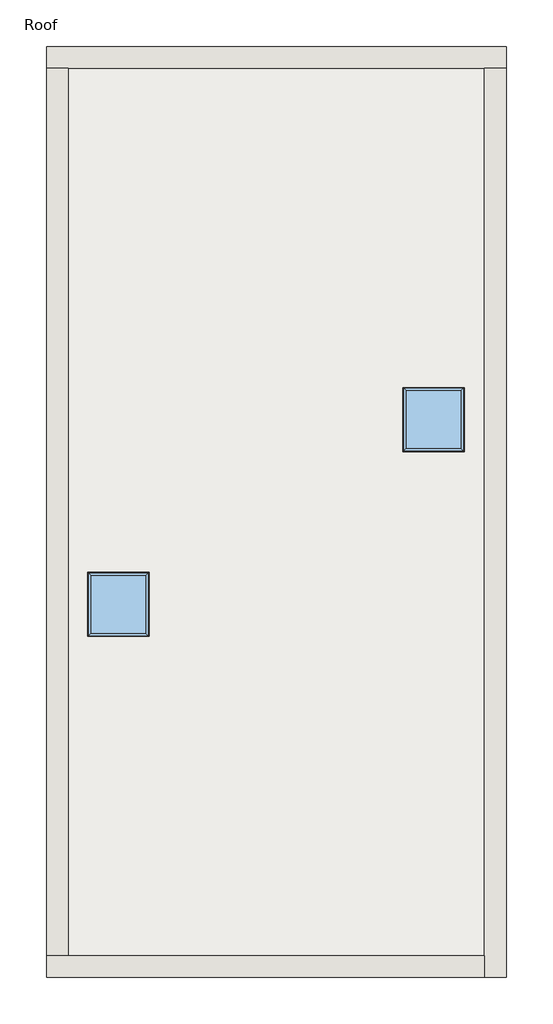
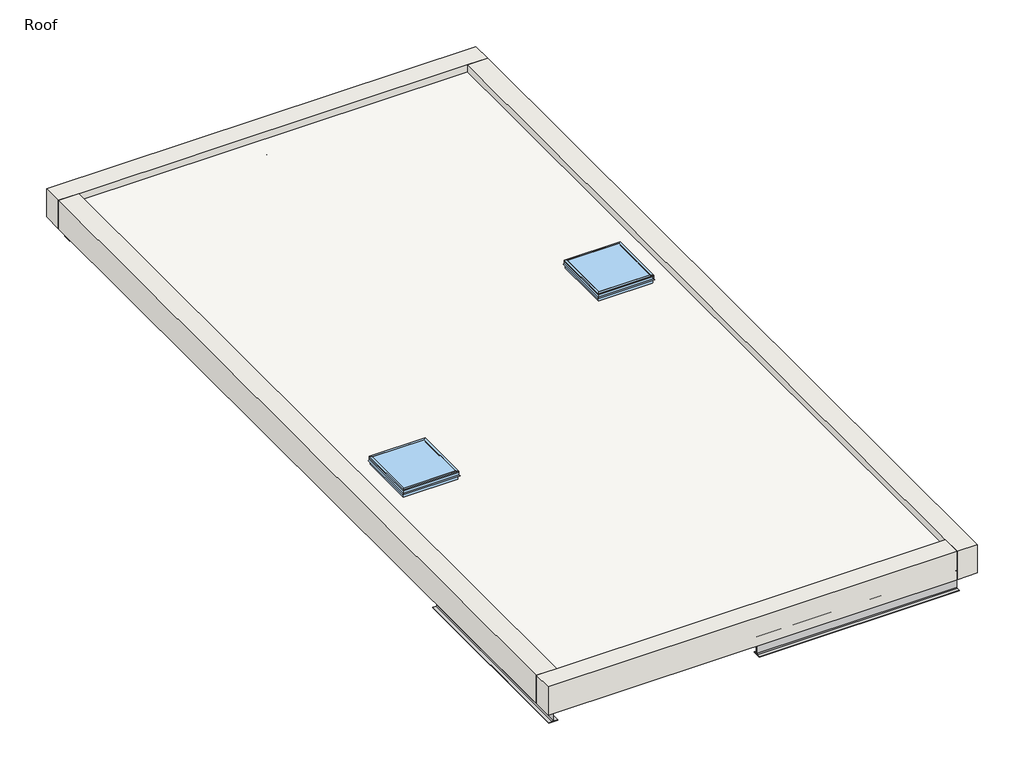
# One storey: 4 beams, 4 walls, 2 windows, 1 roof.
"""IFC4 building model written with IfcOpenShell, lengths in millimetres."""

import ifcopenshell
import ifcopenshell.guid

model = None  # the IFC model being written
_history = None  # IfcOwnerHistory: only IFC2X3 demands one
_inside = {}  # id of a spatial element -> (the spatial element, [elements in it])
_under = {}  # id of a project, library or spatial element -> (it, [spatial elements below it])
_declared = {}  # id of a project -> (the project, [libraries it declares])
_typed = {}  # id of a type object -> (the type object, [elements of that type])
_made_of = {}  # id of a material, layer set ... -> (it, [elements and type objects made of it])


def new_model(schema):
    """Start an empty IFC model of exactly this schema.

    Asked for "IFC4X3", IfcOpenShell would pick the latest addendum, in which some entities
    have other attributes; the version numbers below select the first issue.
    IFC2X3 requires an IfcOwnerHistory on every rooted entity: one is made here for all.
    """
    global model, _history
    if schema == "IFC4X3":
        model = ifcopenshell.file(schema_version=(4, 3, 0, 0))
    else:
        model = ifcopenshell.file(schema=schema)
    _inside.clear()
    _under.clear()
    _declared.clear()
    _typed.clear()
    _made_of.clear()
    _history = None
    if model.schema == "IFC2X3":
        org = make("IfcOrganization", Name="unknown")
        user = make(
            "IfcPersonAndOrganization",
            ThePerson=make("IfcPerson", FamilyName="unknown"),
            TheOrganization=org,
        )
        app = make(
            "IfcApplication",
            ApplicationDeveloper=org,
            Version="unknown",
            ApplicationFullName="unknown",
            ApplicationIdentifier="unknown",
        )
        _history = make(
            "IfcOwnerHistory",
            OwningUser=user,
            OwningApplication=app,
            ChangeAction="ADDED",
            CreationDate=0,
        )
    return model


def make(cls, **values):
    """One entity of the class cls with the attributes given. An attribute that is None is left unset."""
    return model.create_entity(
        cls, **{name: value for name, value in values.items() if value is not None}
    )


def rooted(cls, **values):
    """An entity with a GlobalId (a new one), such as an element, a storey or a relation."""
    return make(cls, GlobalId=ifcopenshell.guid.new(), OwnerHistory=_history, **values)


def si_unit(unit_type, name, prefix=None):
    """IfcSIUnit, for example si_unit("LENGTHUNIT", "METRE", prefix="MILLI")."""
    return make("IfcSIUnit", UnitType=unit_type, Prefix=prefix, Name=name)


def assignment(units):
    """IfcUnitAssignment: the units of a project."""
    return None if units is None else make("IfcUnitAssignment", Units=units)


def point(xyz):
    """IfcCartesianPoint."""
    return None if xyz is None else make("IfcCartesianPoint", Coordinates=xyz)


def direction(xyz):
    """IfcDirection."""
    return None if xyz is None else make("IfcDirection", DirectionRatios=xyz)


def frame(location, z_axis=None, x_axis=None):
    """IfcAxis2Placement3D, a coordinate frame: its origin and axes. An axis left out is left unset."""
    return make(
        "IfcAxis2Placement3D",
        Location=point(location),
        Axis=direction(z_axis),
        RefDirection=direction(x_axis),
    )


def frame_2d(location, x_axis=None):
    """IfcAxis2Placement2D, a coordinate frame in the plane: its origin and x axis."""
    return make(
        "IfcAxis2Placement2D", Location=point(location), RefDirection=direction(x_axis)
    )


def origin():
    """The frame at (0, 0, 0) with its axes left unset."""
    return frame((0.0, 0.0, 0.0))


def place(relative_to, where):
    """IfcLocalPlacement: puts the frame where relative to a parent placement (None: the world)."""
    return make(
        "IfcLocalPlacement", PlacementRelTo=relative_to, RelativePlacement=where
    )


def context(
    kind, dimensions, precision=None, world=None, true_north=None, identifier=None
):
    """IfcGeometricRepresentationContext, for example the 3D "Model" context."""
    return make(
        "IfcGeometricRepresentationContext",
        ContextIdentifier=identifier,
        ContextType=kind,
        CoordinateSpaceDimension=dimensions,
        Precision=precision,
        WorldCoordinateSystem=world,
        TrueNorth=true_north,
    )


def project(units=None, contexts=None):
    """IfcProject with its units and contexts."""
    return rooted(
        "IfcProject",
        Name="project",
        RepresentationContexts=contexts,
        UnitsInContext=assignment(units),
    )


def spatial(cls, under=None, at=None, **own):
    """A site, building, storey or space (cls), placed at a placement, below another one or the project."""
    s = rooted(cls, ObjectPlacement=at, **own)
    if under is not None:
        _under.setdefault(under.id(), (under, []))[1].append(s)
    return s


def polyline(points):
    """IfcPolyline through the points."""
    return make("IfcPolyline", Points=[point(p) for p in points])


def circle_curve(where, radius):
    """IfcCircle in the frame where."""
    return make("IfcCircle", Position=where, Radius=radius)


def trimmed(basis, trim1, trim2, sense, master):
    """IfcTrimmedCurve: the piece of a basis curve between two trims."""
    return make(
        "IfcTrimmedCurve",
        BasisCurve=basis,
        Trim1=trim1,
        Trim2=trim2,
        SenseAgreement=sense,
        MasterRepresentation=master,
    )


def segment(curve, same_sense, transition):
    """IfcCompositeCurveSegment."""
    return make(
        "IfcCompositeCurveSegment",
        Transition=transition,
        SameSense=same_sense,
        ParentCurve=curve,
    )


def composite_curve(segments, self_intersect=None):
    """IfcCompositeCurve: segments joined end to end."""
    return make("IfcCompositeCurve", Segments=segments, SelfIntersect=self_intersect)


def outline(outer, holes=None, kind="AREA"):
    """IfcArbitraryClosedProfileDef: a profile drawn as a closed curve; with holes, ...WithVoids."""
    if holes is None:
        return make("IfcArbitraryClosedProfileDef", ProfileType=kind, OuterCurve=outer)
    return make(
        "IfcArbitraryProfileDefWithVoids",
        ProfileType=kind,
        OuterCurve=outer,
        InnerCurves=holes,
    )


def extrude(swept, where, along, depth):
    """IfcExtrudedAreaSolid: the profile swept, set in the frame where, extruded along a direction by depth."""
    return make(
        "IfcExtrudedAreaSolid",
        SweptArea=swept,
        Position=where,
        ExtrudedDirection=direction(along),
        Depth=depth,
    )


def faces_of(points, faces, orient=None, outer=None):
    """IfcFace entities. A face is a list of loops; a loop is a list of indices into points, from 0.

    orient and outer hold one flag for each loop. By default every Orientation is true, the
    first loop of a face is its IfcFaceOuterBound and the others are IfcFaceBound.
    """
    made = []
    for i, loops in enumerate(faces):
        bounds = []
        for j, loop in enumerate(loops):
            is_outer = j == 0 if outer is None else outer[i][j]
            bounds.append(
                make(
                    "IfcFaceOuterBound" if is_outer else "IfcFaceBound",
                    Bound=make("IfcPolyLoop", Polygon=[points[k] for k in loop]),
                    Orientation=True if orient is None else orient[i][j],
                )
            )
        made.append(make("IfcFace", Bounds=bounds))
    return made


def faceted_brep(points, faces, orient=None, outer=None, voids=None):
    """IfcFacetedBrep: a solid bounded by flat faces; with voids (closed shells), ...WithVoids."""
    shared = [point(p) for p in points]
    hull = make("IfcClosedShell", CfsFaces=faces_of(shared, faces, orient, outer))
    if voids is None:
        return make("IfcFacetedBrep", Outer=hull)
    return make(
        "IfcFacetedBrepWithVoids",
        Outer=hull,
        Voids=[
            make(cls, CfsFaces=faces_of(shared, fs, o, b)) for cls, fs, o, b in voids
        ],
    )


def shape(context_of_items, identifier, shape_type, items):
    """IfcShapeRepresentation: the items that make up one representation, for example the "Body"."""
    return make(
        "IfcShapeRepresentation",
        ContextOfItems=context_of_items,
        RepresentationIdentifier=identifier,
        RepresentationType=shape_type,
        Items=items,
    )


def source(mapping_origin, context_of_items, identifier, shape_type, items):
    """IfcRepresentationMap: a shape defined once, which mapped items show again and again."""
    return make(
        "IfcRepresentationMap",
        MappingOrigin=mapping_origin,
        MappedRepresentation=shape(context_of_items, identifier, shape_type, items),
    )


def transform(
    local_origin,
    x_axis=None,
    y_axis=None,
    z_axis=None,
    scale=None,
    scale2=None,
    scale3=None,
    uniform=True,
):
    """IfcCartesianTransformationOperator3D, or its non-uniform kind. x_axis, y_axis, z_axis: its Axis1, 2, 3."""
    if uniform:
        return make(
            "IfcCartesianTransformationOperator3D",
            Axis1=direction(x_axis),
            Axis2=direction(y_axis),
            LocalOrigin=point(local_origin),
            Scale=scale,
            Axis3=direction(z_axis),
        )
    return make(
        "IfcCartesianTransformationOperator3DnonUniform",
        Axis1=direction(x_axis),
        Axis2=direction(y_axis),
        LocalOrigin=point(local_origin),
        Scale=scale,
        Axis3=direction(z_axis),
        Scale2=scale2,
        Scale3=scale3,
    )


def mapped(mapping_source, mapping_target):
    """IfcMappedItem: shows the shape of a source again, moved by a transform."""
    return make(
        "IfcMappedItem", MappingSource=mapping_source, MappingTarget=mapping_target
    )


def made_of(thing, what):
    """Note that an element or type object is made of a material, layer set ...; save() writes the relation."""
    if what is not None:
        _made_of.setdefault(what.id(), (what, []))[1].append(thing)
    return thing


def element(
    cls,
    number,
    at=None,
    inside=None,
    cuts=None,
    type_object=None,
    material=None,
    context=None,
    identifier="Body",
    shape_type=None,
    held_by="IfcProductDefinitionShape",
    body=None,
    shapes=None,
    **own,
):
    """One element of the class cls, such as IfcWall. Its Tag is "e" and its number.

    at: its placement. inside: the storey or other place that contains it. cuts: it is an
    opening in that element (IfcRelVoidsElement). A single representation is given by context,
    identifier, shape_type and body (its items); several are given by shapes. held_by: the class
    of the entity that holds the representations. save() writes the other relations.
    """
    e = rooted(cls, Tag="e%d" % number, ObjectPlacement=at, **own)
    if body is not None:
        shapes = [shape(context, identifier, shape_type, body)]
    if shapes is not None:
        e.Representation = make(held_by, Representations=shapes)
    if inside is not None:
        _inside.setdefault(inside.id(), (inside, []))[1].append(e)
    if cuts is not None:
        rooted(
            "IfcRelVoidsElement", RelatingBuildingElement=cuts, RelatedOpeningElement=e
        )
    if type_object is not None:
        _typed.setdefault(type_object.id(), (type_object, []))[1].append(e)
    return made_of(e, material)


def aggregate(whole, parts):
    """IfcRelAggregates: a whole, such as a stair, and the parts it consists of."""
    return rooted("IfcRelAggregates", RelatingObject=whole, RelatedObjects=parts)


def save(model, path):
    """Write the relations noted so far, then the file.

    IfcRelAggregates (storeys below a building ...), IfcRelContainedInSpatialStructure (elements
    in a storey), IfcRelDefinesByType, IfcRelAssociatesMaterial and IfcRelDeclares: one each for
    every whole, place, type object, material and project.
    """
    for whole, parts in _under.values():
        aggregate(whole, parts)
    for where, things in _inside.values():
        rooted(
            "IfcRelContainedInSpatialStructure",
            RelatedElements=things,
            RelatingStructure=where,
        )
    for kind, things in _typed.values():
        rooted("IfcRelDefinesByType", RelatedObjects=things, RelatingType=kind)
    for what, things in _made_of.values():
        rooted("IfcRelAssociatesMaterial", RelatedObjects=things, RelatingMaterial=what)
    for by, libraries in _declared.values():
        rooted("IfcRelDeclares", RelatingContext=by, RelatedDefinitions=libraries)
    model.write(path)


def w410x60_ca7ba955(model_context):
    return source(origin(), model_context, "Body", "SweptSolid", [
        extrude(outline(composite_curve([segment(polyline([(89.0, -190.7), (89.0, -203.5), (-89.0, -203.5), (-89.0, -190.7), (-21.05, -190.7)]), True, "CONTINUOUS"), segment(trimmed(circle_curve(frame_2d((-21.05, -173.5)), 17.2), [point((-21.05, -190.7))], [point((-3.85, -173.5))], True, "CARTESIAN"), True, "CONTINUOUS"), segment(polyline([(-3.85, -173.5), (-3.85, 173.5)]), True, "CONTINUOUS"), segment(trimmed(circle_curve(frame_2d((-21.05, 173.5)), 17.2), [point((-3.85, 173.5))], [point((-21.05, 190.7))], True, "CARTESIAN"), True, "CONTINUOUS"), segment(polyline([(-21.05, 190.7), (-89.0, 190.7), (-89.0, 203.5), (89.0, 203.5), (89.0, 190.7), (21.05, 190.7)]), True, "CONTINUOUS"), segment(trimmed(circle_curve(frame_2d((21.05, 173.5)), 17.2), [point((21.05, 190.7))], [point((3.85, 173.5))], True, "CARTESIAN"), True, "CONTINUOUS"), segment(polyline([(3.85, 173.5), (3.85, -173.5)]), True, "CONTINUOUS"), segment(trimmed(circle_curve(frame_2d((21.05, -173.5)), 17.2), [point((3.85, -173.5))], [point((21.05, -190.7))], True, "CARTESIAN"), True, "CONTINUOUS"), segment(polyline([(21.05, -190.7), (89.0, -190.7)]), True, "CONTINUOUS")], self_intersect=False)), frame((-2050.0, 0.0, 0.0), z_axis=(1.0, 0.0, 0.0), x_axis=(0.0, 1.0, 0.0)), (0.0, 0.0, 1.0), 4100.0),
    ])


def w410x60_6fd633e1(model_context):
    return source(origin(), model_context, "Body", "SweptSolid", [
        extrude(outline(composite_curve([segment(polyline([(89.0, -190.7), (89.0, -203.5), (-89.0, -203.5), (-89.0, -190.7), (-21.05, -190.7)]), True, "CONTINUOUS"), segment(trimmed(circle_curve(frame_2d((-21.05, -173.5)), 17.2), [point((-21.05, -190.7))], [point((-3.85, -173.5))], True, "CARTESIAN"), True, "CONTINUOUS"), segment(polyline([(-3.85, -173.5), (-3.85, 173.5)]), True, "CONTINUOUS"), segment(trimmed(circle_curve(frame_2d((-21.05, 173.5)), 17.2), [point((-3.85, 173.5))], [point((-21.05, 190.7))], True, "CARTESIAN"), True, "CONTINUOUS"), segment(polyline([(-21.05, 190.7), (-89.0, 190.7), (-89.0, 203.5), (89.0, 203.5), (89.0, 190.7), (21.05, 190.7)]), True, "CONTINUOUS"), segment(trimmed(circle_curve(frame_2d((21.05, 173.5)), 17.2), [point((21.05, 190.7))], [point((3.85, 173.5))], True, "CARTESIAN"), True, "CONTINUOUS"), segment(polyline([(3.85, 173.5), (3.85, -173.5)]), True, "CONTINUOUS"), segment(trimmed(circle_curve(frame_2d((21.05, -173.5)), 17.2), [point((3.85, -173.5))], [point((21.05, -190.7))], True, "CARTESIAN"), True, "CONTINUOUS"), segment(polyline([(21.05, -190.7), (89.0, -190.7)]), True, "CONTINUOUS")], self_intersect=False)), frame((-2060.6399643, 0.0, 0.0), z_axis=(1.0, 0.0, 0.0), x_axis=(0.0, 1.0, 0.0)), (0.0, 0.0, 1.0), 4121.2799286),
    ])


def m_skylight_1180_x_1170mm_371bb450(model_context):
    return source(origin(), model_context, "Body", "SolidModel", [
        faceted_brep([(254.440073, 370.1040988, 4267.0), (279.840073, 395.5040988, 4267.0), (279.840073, -774.4959012, 4267.0), (254.440073, -749.0959012, 4267.0), (254.440073, 370.1040988, 4292.4), (254.440073, -749.0959012, 4292.4), (292.540073, 408.2040988, 4292.4), (292.540073, -787.1959012, 4292.4), (292.540073, 408.2040988, 4267.0), (292.540073, -787.1959012, 4267.0), (292.540073, 408.2040988, 4216.2), (292.540073, -787.1959012, 4216.2), (307.1089145, 422.7729403, 4195.3935381), (307.1089145, -801.7647427, 4195.3935381), (301.907299, 417.5713248, 4191.7513277), (301.907299, -796.5631272, 4191.7513277), (286.190073, 401.8540988, 4214.1978527), (286.190073, -780.8459012, 4214.1978527), (286.190073, 401.8540988, 4267.0), (286.190073, -780.8459012, 4267.0), (-838.159927, -774.4959012, 4267.0), (-812.759927, -749.0959012, 4267.0), (-812.759927, -749.0959012, 4292.4), (-850.859927, -787.1959012, 4292.4), (-850.859927, -787.1959012, 4267.0), (-850.859927, -787.1959012, 4216.2), (-865.4287685, -801.7647427, 4195.3935381), (-860.227153, -796.5631272, 4191.7513277), (-844.509927, -780.8459012, 4214.1978527), (-844.509927, -780.8459012, 4267.0), (-838.159927, 395.5040988, 4267.0), (-812.759927, 370.1040988, 4267.0), (-812.759927, 370.1040988, 4292.4), (-850.859927, 408.2040988, 4292.4), (-850.859927, 408.2040988, 4267.0), (-850.859927, 408.2040988, 4216.2), (-865.4287685, 422.7729403, 4195.3935381), (-860.227153, 417.5713248, 4191.7513277), (-844.509927, 401.8540988, 4214.1978527), (-844.509927, 401.8540988, 4267.0)], [[[0, 1, 2, 3]], [[4, 0, 3, 5]], [[6, 4, 5, 7]], [[8, 6, 7, 9]], [[10, 8, 9, 11]], [[12, 10, 11, 13]], [[14, 12, 13, 15]], [[16, 14, 15, 17]], [[18, 16, 17, 19]], [[1, 18, 19, 2]], [[3, 2, 20, 21]], [[5, 3, 21, 22]], [[7, 5, 22, 23]], [[9, 7, 23, 24]], [[11, 9, 24, 25]], [[13, 11, 25, 26]], [[15, 13, 26, 27]], [[17, 15, 27, 28]], [[19, 17, 28, 29]], [[2, 19, 29, 20]], [[21, 20, 30, 31]], [[22, 21, 31, 32]], [[23, 22, 32, 33]], [[24, 23, 33, 34]], [[25, 24, 34, 35]], [[26, 25, 35, 36]], [[27, 26, 36, 37]], [[28, 27, 37, 38]], [[29, 28, 38, 39]], [[20, 29, 39, 30]], [[31, 30, 1, 0]], [[32, 31, 0, 4]], [[33, 32, 4, 6]], [[34, 33, 6, 8]], [[35, 34, 8, 10]], [[36, 35, 10, 12]], [[37, 36, 12, 14]], [[38, 37, 14, 16]], [[39, 38, 16, 18]], [[30, 39, 18, 1]]]),
        faceted_brep([(279.840073, -774.4959012, 4267.0), (279.840073, -774.4959012, 4114.6), (279.840073, 395.5040988, 4114.6), (279.840073, 395.5040988, 4267.0), (254.440073, -749.0959012, 4267.0), (254.440073, 370.1040988, 4267.0), (254.440073, -749.0959012, 4241.6), (254.440073, 370.1040988, 4241.6), (235.390073, -730.0459012, 4241.6), (235.390073, 351.0540988, 4241.6), (235.390073, -730.0459012, 4114.6), (235.390073, 351.0540988, 4114.6), (-838.159927, 395.5040988, 4114.6), (-838.159927, 395.5040988, 4267.0), (-812.759927, 370.1040988, 4267.0), (-812.759927, 370.1040988, 4241.6), (-793.709927, 351.0540988, 4241.6), (-793.709927, 351.0540988, 4114.6), (-838.159927, -774.4959012, 4114.6), (-838.159927, -774.4959012, 4267.0), (-812.759927, -749.0959012, 4267.0), (-812.759927, -749.0959012, 4241.6), (-793.709927, -730.0459012, 4241.6), (-793.709927, -730.0459012, 4114.6)], [[[0, 1, 2, 3]], [[4, 0, 3, 5]], [[6, 4, 5, 7]], [[8, 6, 7, 9]], [[10, 8, 9, 11]], [[1, 10, 11, 2]], [[3, 2, 12, 13]], [[5, 3, 13, 14]], [[7, 5, 14, 15]], [[9, 7, 15, 16]], [[11, 9, 16, 17]], [[2, 11, 17, 12]], [[13, 12, 18, 19]], [[14, 13, 19, 20]], [[15, 14, 20, 21]], [[16, 15, 21, 22]], [[17, 16, 22, 23]], [[12, 17, 23, 18]], [[19, 18, 1, 0]], [[20, 19, 0, 4]], [[21, 20, 4, 6]], [[22, 21, 6, 8]], [[23, 22, 8, 10]], [[18, 23, 10, 1]]]),
        extrude(outline(polyline([(254.440073, -749.0959012), (-812.759927, -749.0959012), (-812.759927, 370.1040988), (254.440073, 370.1040988), (254.440073, -749.0959012)])), frame((0.0, 0.0, 4286.05), z_axis=(0.0, 0.0, 1.0), x_axis=(1.0, 0.0, 0.0)), (0.0, 0.0, 1.0), 6.35),
    ])


model = new_model("IFC4")

# Units and contexts
model_context = context("Model", 3, world=origin())
ifc_project = project(units=[si_unit("LENGTHUNIT", "METRE", prefix="MILLI")], contexts=[model_context])

# Site, building, storey
site = spatial("IfcSite", under=ifc_project)
building = spatial("IfcBuilding", under=site)
storey = spatial("IfcBuildingStorey", under=building, Name="Roof", Elevation=6000.0)

# Beams
placement = place(None, origin())
w410x60_shape = w410x60_ca7ba955(model_context)
element("IfcBeam", 1, ObjectType="M_W-Wide Flange : W410X60", at=placement, inside=storey, context=model_context, shape_type="MappedRepresentation", body=[
    mapped(w410x60_shape, transform((6478.9543287, -17528.766863, 5796.5), x_axis=(1.0, 0.0, 0.0), y_axis=(0.0, 1.0, 0.0), z_axis=(0.0, 0.0, 1.0))),
])
element("IfcBeam", 2, ObjectType="M_W-Wide Flange : W410X60", at=placement, inside=storey, context=model_context, shape_type="MappedRepresentation", body=[
    mapped(w410x60_shape, transform((2321.0456713, -271.233137, 5796.5), x_axis=(-1.0, 0.0, 0.0), y_axis=(0.0, -1.0, 0.0), z_axis=(0.0, 0.0, 1.0))),
])
w410x60_2_shape = w410x60_6fd633e1(model_context)
element("IfcBeam", 3, ObjectType="M_W-Wide Flange : W410X60", at=placement, inside=storey, context=model_context, shape_type="MappedRepresentation", body=[
    mapped(w410x60_2_shape, transform((266.6128796, -15462.3600357, 5796.5), x_axis=(0.0, -1.0, 0.0), y_axis=(1.0, 0.0, 0.0), z_axis=(0.0, 0.0, 1.0))),
])
element("IfcBeam", 4, ObjectType="M_W-Wide Flange : W410X60", at=placement, inside=storey, context=model_context, shape_type="MappedRepresentation", body=[
    mapped(w410x60_2_shape, transform((8533.3871204, -2337.6399643, 5796.5), x_axis=(0.0, 1.0, 0.0), y_axis=(-1.0, 0.0, 0.0), z_axis=(0.0, 0.0, 1.0))),
])

# Roof
element("IfcRoof", 5, ObjectType="Live Roof over Wood Joist Flat Roof", at=placement, inside=storey, context=model_context, shape_type="SweptSolid", body=[
    extrude(outline(polyline([(417.0, -417.0), (8383.0, -417.0), (8383.0, -17383.0), (417.0, -17383.0), (417.0, -417.0)]), holes=[polyline([(1890.55, -10124.45), (861.45, -10124.45), (861.45, -11205.55), (1890.55, -11205.55), (1890.55, -10124.45)]), polyline([(7923.55, -6594.45), (6894.45, -6594.45), (6894.45, -7675.55), (7923.55, -7675.55), (7923.55, -6594.45)])]), frame((0.0, 0.0, 6000.0), z_axis=(0.0, 0.0, 1.0), x_axis=(1.0, 0.0, 0.0)), (0.0, 0.0, 1.0), 457.0),
])

# Walls
element("IfcWall", 6, ObjectType="Exterior - Brick on Block", at=placement, inside=storey, context=model_context, shape_type="Brep", body=[
    faceted_brep([(0.0, -417.0, 6000.0), (417.0, -417.0, 6000.0), (8383.0, -417.0, 6000.0), (8800.0, -417.0, 6000.0), (8800.0, -417.0, 6609.0), (8383.0, -417.0, 6609.0), (417.0, -417.0, 6609.0), (0.0, -417.0, 6609.0), (0.0, 0.0, 6000.0), (0.0, 0.0, 6609.0), (8800.0, 0.0, 6609.0), (8800.0, 0.0, 6000.0)], [[[0, 1, 2, 3, 4, 5, 6, 7]], [[8, 9, 10, 11]], [[3, 2, 1, 0, 8, 11]], [[7, 6, 5, 4, 10, 9]], [[4, 3, 11, 10]], [[0, 7, 9, 8]]]),
])
element("IfcWall", 7, ObjectType="Exterior - Brick on Block", at=placement, inside=storey, context=model_context, shape_type="Brep", body=[
    faceted_brep([(8383.0, -417.0, 6000.0), (8383.0, -17383.0, 6000.0), (8383.0, -17800.0, 6000.0), (8383.0, -17800.0, 6609.0), (8383.0, -17383.0, 6609.0), (8383.0, -417.0, 6609.0), (8800.0, -417.0, 6000.0), (8800.0, -417.0, 6609.0), (8800.0, -17800.0, 6609.0), (8800.0, -17800.0, 6000.0)], [[[0, 1, 2, 3, 4, 5]], [[6, 7, 8, 9]], [[2, 1, 0, 6, 9]], [[5, 4, 3, 8, 7]], [[0, 5, 7, 6]], [[3, 2, 9, 8]]]),
])
element("IfcWall", 8, ObjectType="Exterior - Brick on Block", at=placement, inside=storey, context=model_context, shape_type="Brep", body=[
    faceted_brep([(8383.0, -17383.0, 6000.0), (417.0, -17383.0, 6000.0), (0.0, -17383.0, 6000.0), (0.0, -17383.0, 6609.0), (417.0, -17383.0, 6609.0), (8383.0, -17383.0, 6609.0), (8383.0, -17800.0, 6000.0), (8383.0, -17800.0, 6609.0), (0.0, -17800.0, 6609.0), (0.0, -17800.0, 6000.0)], [[[0, 1, 2, 3, 4, 5]], [[6, 7, 8, 9]], [[2, 1, 0, 6, 9]], [[5, 4, 3, 8, 7]], [[0, 5, 7, 6]], [[3, 2, 9, 8]]]),
])
element("IfcWall", 9, ObjectType="Exterior - Brick on Block", at=placement, inside=storey, context=model_context, shape_type="SweptSolid", body=[
    extrude(outline(polyline([(417.0, -417.0), (417.0, -17383.0), (0.0, -17383.0), (0.0, -417.0), (417.0, -417.0)])), frame((0.0, 0.0, 6000.0), z_axis=(0.0, 0.0, 1.0), x_axis=(1.0, 0.0, 0.0)), (0.0, 0.0, 1.0), 609.0),
])

# Windows
m_skylight_1180_x_1170mm_shape = m_skylight_1180_x_1170mm_371bb450(model_context)
element("IfcWindow", 10, ObjectType="M_Skylight : 1180 x 1170mm", at=placement, inside=storey, context=model_context, shape_type="MappedRepresentation", body=[
    mapped(m_skylight_1180_x_1170mm_shape, transform((1655.159927, -10475.5040988, 2342.4), x_axis=(1.0, 0.0, 0.0), y_axis=(0.0, 1.0, 0.0), z_axis=(0.0, 0.0, 1.0))),
])
element("IfcWindow", 11, ObjectType="M_Skylight : 1180 x 1170mm", at=placement, inside=storey, context=model_context, shape_type="MappedRepresentation", body=[
    mapped(m_skylight_1180_x_1170mm_shape, transform((7688.159927, -6945.5040988, 2342.4), x_axis=(1.0, 0.0, 0.0), y_axis=(0.0, 1.0, 0.0), z_axis=(0.0, 0.0, 1.0))),
])

save(model, "model.ifc")

# Revit data of these elements
# Type "M_W-Wide Flange : W410X60"
#   Manufacturer = "Manufacturer"
#   AccessibilityPerformance = "AccessibilityPerformance"
#   CodePerformance = "CodePerformance"
#   Color = "Color"
#   Constituents = "Constituents"
#   Features = "Features"
#   Finish = "Finish"
#   Grade = "Grade"
#   Material = "Material"
#   ModelReference = "ModelReference"
#   NominalHeight = "NominalHeight"
#   NominalLength = "NominalLength"
#   NominalWidth = "NominalWidth"
#   ProductionYear = "ProductionYear"
#   Reference = "Reference"
#   Shape = "Shape"
#   Size = "Size"
#   SustainabilityPerformance = "SustainabilityPerformance"
#   WarrantyDescription = "WarrantyDescription"
#   WarrantyDurationLabor = "WarrantyDurationLabor"
#   WarrantyDurationParts = "WarrantyDurationParts"
#   WarrantyGuarantorLabor = "WarrantyGuarantorLabor"
#   WarrantyGuarantorParts = "WarrantyGuarantorParts"
#   ExpectedLife = "ExpectedLife"
#   ReplacementCost = "ReplacementCost"
#   AssetAccountingType = "FIXED"
#   ModelLabel = "ModelLabel"
#   W = 0.58
#   Start Extension Calculation [instance default] = 3.000 m
#   Start Extension [instance default] = -0.0127 m
#   End Extension Calculation [instance default] = 3.000 m
#   End Extension [instance default] = -0.0127 m
#   Length [instance default] = 1.524 m
#   bf = 0.178 m
#   d = 0.407 m
#   k = 0.030 m
#   kr = 0.0172 m
#   tf = 0.0128 m
#   tw = 0.0077 m
#   A = 0.0076 m²
#   Structural Material [instance default] = Metal - Steel - 345 MPa
#   Assembly Code = ""
# Type "Live Roof over Wood Joist Flat Roof"
#   Manufacturer = "Manufacturer"
#   AccessibilityPerformance = "AccessibilityPerformance"
#   CodePerformance = "CodePerformance"
#   Color = "Color"
#   Constituents = "Constituents"
#   Features = "Features"
#   Finish = "Finish"
#   Grade = "Grade"
#   Material = "Material"
#   ModelReference = "ModelReference"
#   NominalHeight = "NominalHeight"
#   NominalLength = "NominalLength"
#   NominalWidth = "NominalWidth"
#   ProductionYear = "ProductionYear"
#   Reference = "Reference"
#   Shape = "Shape"
#   Size = "Size"
#   SustainabilityPerformance = "SustainabilityPerformance"
#   WarrantyDescription = "WarrantyDescription"
#   WarrantyDurationLabor = "WarrantyDurationLabor"
#   WarrantyDurationParts = "WarrantyDurationParts"
#   WarrantyGuarantorLabor = "WarrantyGuarantorLabor"
#   WarrantyGuarantorParts = "WarrantyGuarantorParts"
#   ExpectedLife = "ExpectedLife"
#   ReplacementCost = "ReplacementCost"
#   AssetAccountingType = "FIXED"
#   Classification Description = "Structural Roof Decks"
#   Classification Code = "23-25 30 27 14"
#   ModelLabel = "ModelLabel"
#   Layers, outside or top first: 0.064 m "Site - Grass" (function 5); 0.006 m "Roofing - Barrier" (function 4); 0.006 m "Roofing - EPDM Membrane" (function 4); 0.076 m "Insulation / Thermal Barriers - Rigid insulation" (function 3); 0.019 m "Wood - Sheathing - plywood" (function 2); 0.286 m "Wood - Dimensional Lumber" (function 1)
# Type "Exterior - Brick on Block"
#   Manufacturer = "Manufacturer"
#   AccessibilityPerformance = "AccessibilityPerformance"
#   CodePerformance = "CodePerformance"
#   Color = "Color"
#   Constituents = "Constituents"
#   Features = "Features"
#   Finish = "Finish"
#   Grade = "Grade"
#   Material = "Material"
#   ModelReference = "ModelReference"
#   NominalHeight = "NominalHeight"
#   NominalLength = "NominalLength"
#   NominalWidth = "NominalWidth"
#   ProductionYear = "ProductionYear"
#   Reference = "Reference"
#   Shape = "Shape"
#   Size = "Size"
#   SustainabilityPerformance = "SustainabilityPerformance"
#   WarrantyDescription = "WarrantyDescription"
#   WarrantyDurationLabor = "WarrantyDurationLabor"
#   WarrantyDurationParts = "WarrantyDurationParts"
#   WarrantyGuarantorLabor = "WarrantyGuarantorLabor"
#   WarrantyGuarantorParts = "WarrantyGuarantorParts"
#   ExpectedLife = "ExpectedLife"
#   ReplacementCost = "ReplacementCost"
#   AssetAccountingType = "FIXED"
#   Classification Description = "Masonry Structural Walls"
#   Classification Code = "23-25 30 24 14"
#   ModelLabel = "ModelLabel"
#   Layers, outside or top first: 0.092 m "Masonry - Brick" (function 4); 0.025 m "Misc. Air Layers - Air Space" (function 3); 0.000 m "Air Barrier - Air Infiltration Barrier" (function 100); 0.050 m "Insulation / Thermal Barriers - Rigid insulation" (function 3); 0.193 m "Masonry - Concrete Block" (function 1); 0.041 m "Metal - Stud Layer" (function 2); 0.000 m "Vapour / Moisture Barriers - Vapour Retarder" (function 100); 0.016 m "Plasterboard" (function 5)
# Type "M_Skylight : 1180 x 1170mm"
#   Manufacturer = "Manufacturer"
#   Type Mark = "36"
#   Construction Type = "Construction Type"
#   AccessibilityPerformance = "AccessibilityPerformance"
#   CodePerformance = "CodePerformance"
#   ConfigurationType = "ConfigurationType"
#   ConstructionType = "ConstructionType"
#   FireRating = "FireRating"
#   GlazingAreaFraction = "GlazingAreaFraction"
#   OperationType = "OperationType"
#   Area = "Area"
#   Color = "Color"
#   Constituents = "Constituents"
#   Features = "Features"
#   Finish = "Finish"
#   Grade = "Grade"
#   Material = "Material"
#   ModelReference = "ModelReference"
#   NominalHeight = "NominalHeight"
#   NominalLength = "NominalLength"
#   NominalWidth = "NominalWidth"
#   ProductionYear = "ProductionYear"
#   Reference = "Reference"
#   Shape = "Shape"
#   Size = "Size"
#   SustainabilityPerformance = "SustainabilityPerformance"
#   WarrantyDescription = "WarrantyDescription"
#   WarrantyDurationLabor = "WarrantyDurationLabor"
#   WarrantyDurationParts = "WarrantyDurationParts"
#   WarrantyGuarantorLabor = "WarrantyGuarantorLabor"
#   WarrantyGuarantorParts = "WarrantyGuarantorParts"
#   ExpectedLife = "ExpectedLife"
#   ReplacementCost = "ReplacementCost"
#   AssetAccountingType = "FIXED"
#   ModelLabel = "ModelLabel"
#   Height = 1.170 m
#   Width = 1.118 m
#   Sash Material = Metal - Bronze, Light Brush
#   Glass Pane Material = Glass
#   Frame Material = Metal - Bronze, Light Brush
#   Type Comments = ""
# Elements 1, 2, 3, 4 (IfcBeam, "M_W-Wide Flange : W410X60")
#   InstallationDate = "InstallationDate"
#   SerialNumber = "SerialNumber"
#   WarrantyStartDate = "WarrantyStartDate"
#   BarCode = "BarCode"
#   AssetIdentifier = "AssetIdentifier"
#   TagNumber = "TagNumber"
#   Start Extension Calculation = 3.000 m
#   Start Extension = -0.0127 m
#   End Extension Calculation = 3.000 m
#   End Extension = -0.0127 m
#   Structural Material = Metal - Steel - 345 MPa
#   Phase Created = New Construction
#   Materials on its faces: "Metal - Steel - 345 MPa"
# Element 5 (IfcRoof, "Live Roof over Wood Joist Flat Roof")
#   InstallationDate = "InstallationDate"
#   SerialNumber = "SerialNumber"
#   WarrantyStartDate = "WarrantyStartDate"
#   BarCode = "BarCode"
#   AssetIdentifier = "AssetIdentifier"
#   TagNumber = "TagNumber"
#   built-in parameter 1001705 = 21.1844 (stored number, unit not read)
#   built-in parameter 1001710 = 33615
#   Phase Created = New Construction
#   Materials on its faces: "Wood - Dimensional Lumber", "Site - Grass"
# Element 6 (IfcWall, "Exterior - Brick on Block")
#   InstallationDate = "InstallationDate"
#   SerialNumber = "SerialNumber"
#   WarrantyStartDate = "WarrantyStartDate"
#   BarCode = "BarCode"
#   AssetIdentifier = "AssetIdentifier"
#   TagNumber = "TagNumber"
#   URI = "https://niras.dk/projects/0001/wall_1xS3BCk291UvhgP2dvNxPL"
#   Top Offset = 0.609 m
#   Base Offset = 0.000 m
#   wall height = 0.609 m
#   Phase Created = New Construction
#   Base Constraint = Roof
#   Top Constraint = Roof
#   Materials on its faces: "Masonry - Brick", "Default Wall", "Plasterboard"
# Element 7 (IfcWall, "Exterior - Brick on Block")
#   InstallationDate = "InstallationDate"
#   SerialNumber = "SerialNumber"
#   WarrantyStartDate = "WarrantyStartDate"
#   BarCode = "BarCode"
#   AssetIdentifier = "AssetIdentifier"
#   TagNumber = "TagNumber"
#   URI = "https://niras.dk/projects/0001/wall_1xS3BCk291UvhgP2dvNxQJ"
#   Top Offset = 0.609 m
#   Base Offset = 0.000 m
#   wall height = 0.609 m
#   Phase Created = New Construction
#   Base Constraint = Roof
#   Top Constraint = Roof
#   Materials on its faces: "Default Wall", "Masonry - Brick", "Plasterboard"
# Element 8 (IfcWall, "Exterior - Brick on Block")
#   InstallationDate = "InstallationDate"
#   SerialNumber = "SerialNumber"
#   WarrantyStartDate = "WarrantyStartDate"
#   BarCode = "BarCode"
#   AssetIdentifier = "AssetIdentifier"
#   TagNumber = "TagNumber"
#   URI = "https://niras.dk/projects/0001/wall_1xS3BCk291UvhgP2dvNxRD"
#   Top Offset = 0.609 m
#   Base Offset = 0.000 m
#   wall height = 0.609 m
#   Phase Created = New Construction
#   Base Constraint = Roof
#   Top Constraint = Roof
#   Materials on its faces: "Default Wall", "Masonry - Brick", "Plasterboard"
# Element 9 (IfcWall, "Exterior - Brick on Block")
#   InstallationDate = "InstallationDate"
#   SerialNumber = "SerialNumber"
#   WarrantyStartDate = "WarrantyStartDate"
#   BarCode = "BarCode"
#   AssetIdentifier = "AssetIdentifier"
#   TagNumber = "TagNumber"
#   URI = "https://niras.dk/projects/0001/wall_1xS3BCk291UvhgP2dvNxSe"
#   Top Offset = 0.609 m
#   Base Offset = 0.000 m
#   wall height = 0.609 m
#   Phase Created = New Construction
#   Base Constraint = Roof
#   Top Constraint = Roof
#   Materials on its faces: "Default Wall", "Plasterboard", "Masonry - Brick"
# Element 10 (IfcWindow, "M_Skylight : 1180 x 1170mm")
#   Mark = "33"
#   InstallationDate = "InstallationDate"
#   SerialNumber = "SerialNumber"
#   WarrantyStartDate = "WarrantyStartDate"
#   BarCode = "BarCode"
#   AssetIdentifier = "AssetIdentifier"
#   TagNumber = "TagNumber"
#   URI = "https://niras.dk/projects/0001/window_1xS3BCk291UvhgP2dvNxVS"
#   Phase Created = New Construction
#   Materials on its faces: "Metal - Bronze, Light Brush", "Glass"
# Element 11 (IfcWindow, "M_Skylight : 1180 x 1170mm")
#   Mark = "34"
#   InstallationDate = "InstallationDate"
#   SerialNumber = "SerialNumber"
#   WarrantyStartDate = "WarrantyStartDate"
#   BarCode = "BarCode"
#   AssetIdentifier = "AssetIdentifier"
#   TagNumber = "TagNumber"
#   URI = "https://niras.dk/projects/0001/window_1xS3BCk291UvhgP2dvNx5J"
#   Phase Created = New Construction
#   Materials on its faces: "Metal - Bronze, Light Brush", "Glass"
# Materials
#   "Metal - Steel - 345 MPa": class "Metal", colour RGB 247 247 247, transparency 0
#   "Site - Grass": class "Plant", colour RGB 78 100 75, transparency 0
#   "Roofing - Barrier": class "Plastic", colour RGB 127 127 127, transparency 0, Description = "Exterior finish, roofing"
#   "Roofing - EPDM Membrane": class "Plastic", colour RGB 127 127 127, transparency 0, Description = "Exterior finish, roofing"
#   "Insulation / Thermal Barriers - Rigid insulation": class "Miscellaneous", colour RGB 127 127 127, transparency 0
#   "Wood - Sheathing - plywood": class "Wood", colour RGB 184 187 68, transparency 0
#   "Wood - Dimensional Lumber": class "Wood", colour RGB 223 192 134, transparency 0, Cost = 0
#   "Masonry - Brick": class "Brick", colour RGB 170 100 105, transparency 0, Cost = 0
#   "Misc. Air Layers - Air Space": class "Miscellaneous", colour RGB 255 255 255, transparency 0
#   "Air Barrier - Air Infiltration Barrier": class "Miscellaneous", colour RGB 127 127 127, transparency 0
#   "Masonry - Concrete Block": class "Concrete", colour RGB 181 181 181, transparency 0
#   "Metal - Stud Layer": class "Metal", colour RGB 127 127 127, transparency 0
#   "Vapour / Moisture Barriers - Vapour Retarder": class "Miscellaneous", colour RGB 127 127 127, transparency 0
#   "Plasterboard": class "Drywall", colour RGB 249 249 249, transparency 0, Description = "Interior finish"
#   "Metal - Bronze, Light Brush": class "Metal", colour RGB 113 80 70, transparency 0
#   "Glass": class "Glass", colour RGB 0 128 192, transparency 0.9
#   "Default Wall": class "Miscellaneous", colour RGB 128 128 128, transparency 0
# Room at (4700.151, -8954.117) mm, phase "New Construction", upper level "Roof", upper offset 3.000 m, lower offset 0.000 m
#   Number = "R301"
#   Name = "Roof"
#   CeilingCovering = "CeilingCovering"
#   FloorCovering = "FloorCovering"
#   WallCovering = "WallCovering"
#   LoadCapacity = "LoadCapacity"
#   CirculationZoneName = "Roof CirculationZoneName"
#   FireAlarmZoneName = "Roof FireAlarmZoneName"
#   HistoricPreservationZoneName = "Roof HistoricPreservationZoneName"
#   LightingZoneName = "Roof LightingZoneName"
#   OccupancyZoneName = "Roof OccupancyZoneName"
#   VentilationZoneName = "Roof VentilationZoneName"
#   RoomTag = "RoomTag"
#   URI = "https://niras.dk/projects/0001/room_1xS3BCk291UvhgP2dvNbq0"
#   OmniClass Table 13 Category = 13-81 11 99: Other General Facility Service Spaces
